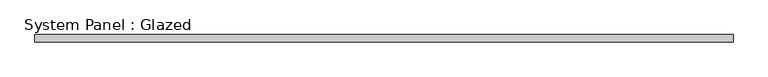
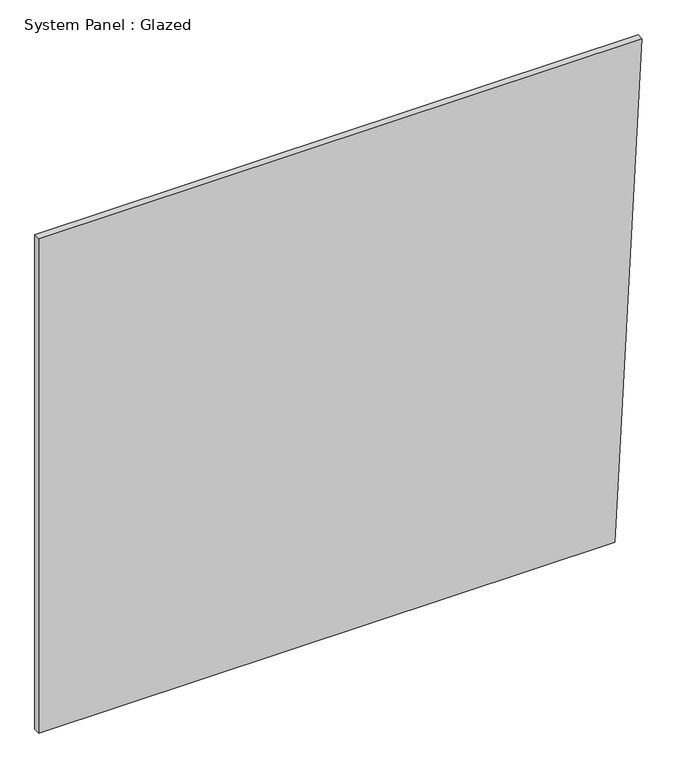
"""IFC4 building model written with IfcOpenShell, lengths in millimetres: plate geometry, System Panel : Glazed."""

from ifc_helpers import new_model, si_unit, frame, origin, place, context, project, spatial, polyline, outline, extrude, source, transform, mapped, element, save


def system_panel_glazed_bfd5517e(model_context):
    return source(origin(), model_context, "Body", "SweptSolid", [
        extrude(outline(polyline([(0.0, -1204.673413), (0.0, 1095.4915598), (2086.1728929, 1204.673413), (2086.1728929, -1204.673413), (0.0, -1204.673413)])), frame((0.0, -44.45, 0.0), z_axis=(0.0, 1.0, 0.0), x_axis=(0.0, 0.0, 1.0)), (0.0, 0.0, 1.0), 25.4),
    ])


if __name__ == "__main__":
    model = new_model("IFC4")
    model_context = context("Model", 3, world=origin())
    ifc_project = project(units=[si_unit("LENGTHUNIT", "METRE", prefix="MILLI")], contexts=[model_context])
    site = spatial("IfcSite", under=ifc_project)
    building = spatial("IfcBuilding", under=site)
    placement = place(None, origin())
    system_panel_glazed_shape = system_panel_glazed_bfd5517e(model_context)
    element("IfcPlate", 1, ObjectType="System Panel : Glazed", at=placement, inside=building, context=model_context, shape_type="MappedRepresentation", body=[
        mapped(system_panel_glazed_shape, transform((0.0, 0.0, 0.0), x_axis=(1.0, 0.0, 0.0), y_axis=(0.0, 1.0, 0.0), z_axis=(0.0, 0.0, 1.0))),
    ])
    save(model, "model.ifc")

# Revit data of these elements
# Type "System Panel : Glazed"
#   Construction Type Id = "GSP4R"
#   Analytic Construction = "1/8 in Pilkington single glazing"
#   Visual Light Transmittance = 0.9
#   Solar Heat Gain Coefficient = 0.86
#   Heat Transfer Coefficient (U) = 1.18115 BTU/(h·ft²·°F)
#   Define Thermal Properties by = 1
# Element 1 (IfcPlate, "System Panel : Glazed")
#   Materials on its faces: "Glass"
# Materials
#   "Glass": class "Glass", colour RGB 0 128 192, transparency 0.75, Description = "Soda Lime Glass", Cost = 0
